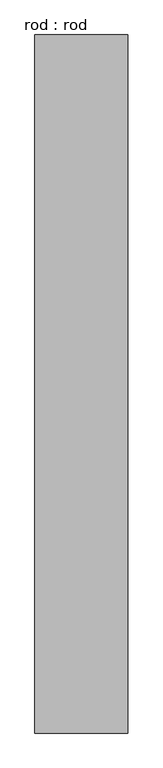
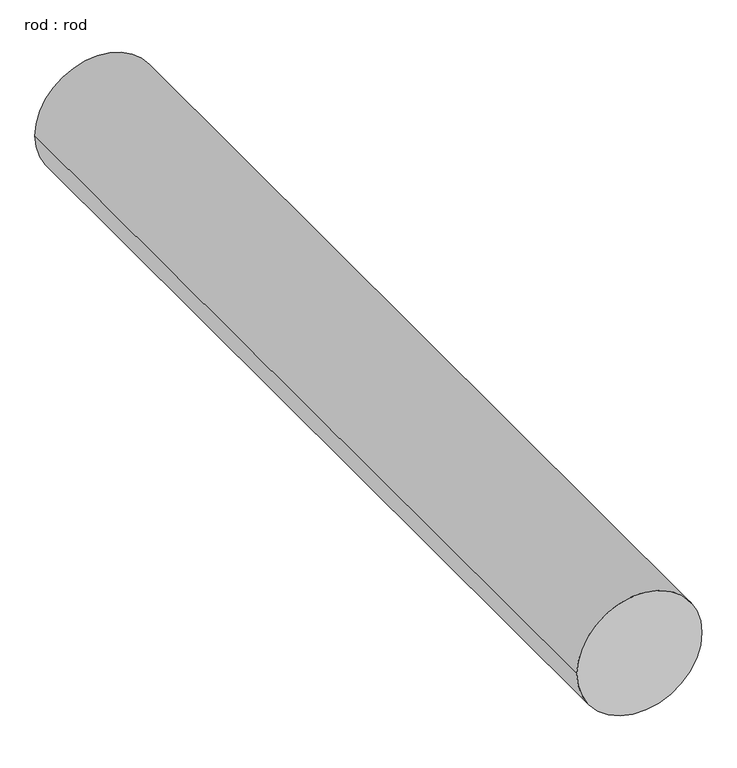
"""IFC4 building model written with IfcOpenShell, lengths in millimetres: proxy geometry, rod : rod."""

from ifc_helpers import new_model, si_unit, point, frame, frame_2d, origin, place, context, project, spatial, circle_curve, trimmed, segment, composite_curve, outline, extrude, source, transform, mapped, element, save


def rod_rod_60cdffe7(model_context):
    return source(origin(), model_context, "Body", "SweptSolid", [
        extrude(outline(composite_curve([segment(trimmed(circle_curve(frame_2d((0.0108462, 0.0)), 200.0), [point((0.0108462, 200.0))], [point((0.0108462, -200.0))], False, "CARTESIAN"), True, "CONTINUOUS"), segment(trimmed(circle_curve(frame_2d((0.0108462, 0.0)), 200.0), [point((0.0108462, -200.0))], [point((0.0108462, 200.0))], False, "CARTESIAN"), True, "CONTINUOUS")], self_intersect=False)), frame((0.0, 2592.7286153, 0.0), z_axis=(0.0, 1.0, 0.0), x_axis=(0.0, 0.0, 1.0)), (0.0, 0.0, 1.0), 3000.0),
    ])


if __name__ == "__main__":
    model = new_model("IFC4")
    model_context = context("Model", 3, world=origin())
    ifc_project = project(units=[si_unit("LENGTHUNIT", "METRE", prefix="MILLI")], contexts=[model_context])
    site = spatial("IfcSite", under=ifc_project)
    building = spatial("IfcBuilding", under=site)
    placement = place(None, origin())
    rod_rod_shape = rod_rod_60cdffe7(model_context)
    element("IfcBuildingElementProxy", 1, Name="rod : rod", ObjectType="rod : rod", at=placement, inside=building, context=model_context, shape_type="MappedRepresentation", body=[
        mapped(rod_rod_shape, transform((0.0, 0.0, 0.0), x_axis=(1.0, 0.0, 0.0), y_axis=(0.0, 1.0, 0.0), z_axis=(0.0, 0.0, 1.0))),
    ])
    save(model, "model.ifc")

# Revit data of these elements
# Type "rod : rod"
#   Default Elevation = 0
